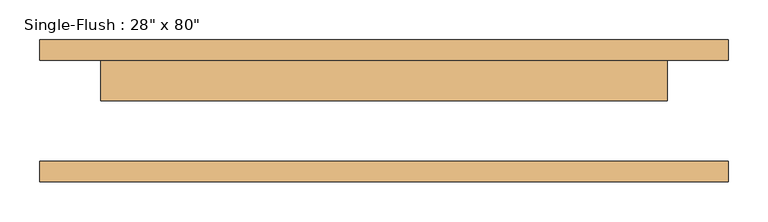
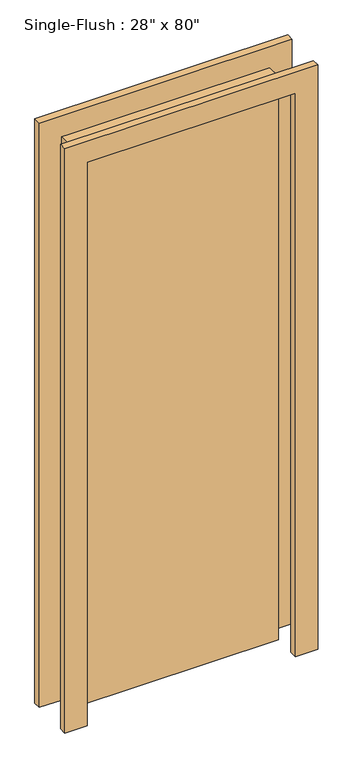
"""IFC4 building model written with IfcOpenShell, lengths in millimetres: door geometry."""

from ifc_helpers import new_model, si_unit, frame, origin, origin_with_axes, place, context, project, spatial, polyline, outline, extrude, source, transform, mapped, element, save


def door_7f94203e(model_context):
    return source(origin(), model_context, "Body", "SweptSolid", [
        extrude(outline(polyline([(2108.2, -431.8), (0.0, -431.8), (0.0, -355.6), (2032.0, -355.6), (2032.0, 355.6), (0.0, 355.6), (0.0, 431.8), (2108.2, 431.8), (2108.2, -431.8)])), frame((0.0, 63.5, 0.0), z_axis=(0.0, 1.0, 0.0), x_axis=(0.0, 0.0, 1.0)), (0.0, 0.0, 1.0), 25.4),
        extrude(outline(polyline([(2108.2, 431.8), (2108.2, -431.8), (0.0, -431.8), (0.0, -355.6), (2032.0, -355.6), (2032.0, 355.6), (0.0, 355.6), (0.0, 431.8), (2108.2, 431.8)])), frame((0.0, -88.9, 0.0), z_axis=(0.0, 1.0, 0.0), x_axis=(0.0, 0.0, 1.0)), (0.0, 0.0, 1.0), 25.4),
        extrude(outline(polyline([(355.6, 12.7), (-355.6, 12.7), (-355.6, 63.5), (355.6, 63.5), (355.6, 12.7)])), origin_with_axes(), (0.0, 0.0, 1.0), 2032.0),
    ])


if __name__ == "__main__":
    model = new_model("IFC4")
    model_context = context("Model", 3, world=origin())
    ifc_project = project(units=[si_unit("LENGTHUNIT", "METRE", prefix="MILLI")], contexts=[model_context])
    site = spatial("IfcSite", under=ifc_project)
    building = spatial("IfcBuilding", under=site)
    placement = place(None, origin())
    door_shape = door_7f94203e(model_context)
    element("IfcDoor", 1, ObjectType="Single-Flush : 28\" x 80\"", at=placement, inside=building, context=model_context, shape_type="MappedRepresentation", body=[
        mapped(door_shape, transform((0.0, 0.0, 0.0), x_axis=(1.0, 0.0, 0.0), y_axis=(0.0, 1.0, 0.0), z_axis=(0.0, 0.0, 1.0))),
    ])
    save(model, "model.ifc")

# Revit data of these elements
# Type "Single-Flush : 28\" x 80\""
#   Type Mark = "13"
#   Construction Type Id = "MDOOR"
#   Assembly Code = "C1020"
#   Analytic Construction = "Metal"
#   Thickness = 0' - 2"
#   Heat Transfer Coefficient (U) = 0.651978 BTU/(h·ft²·°F)
#   Height = 6' - 8"
#   Trim Projection Ext = 0' - 1"
#   Trim Projection Int = 0' - 1"
#   Trim Width = 0' - 3"
#   Width = 2' - 4"
#   Define Thermal Properties by = 1
#   Door Material = Door - Panel
#   Frame Material = Door - Frame
#   Visual Light Transmittance = 0
#   Solar Heat Gain Coefficient = 0
#   Function = (empty or 0)
#   Wall Closure = (empty or 0)
# Element 1 (IfcDoor, "Single-Flush : 28\" x 80\"")
#   Materials on its faces: "Door - Frame", "Door - Panel"
# Materials
#   "Door - Panel": class "Wood", colour RGB 210 159 95, transparency 0, Cost = 0
#   "Door - Frame": class "Miscellaneous", colour RGB 118 70 51, transparency 0, Cost = 0
